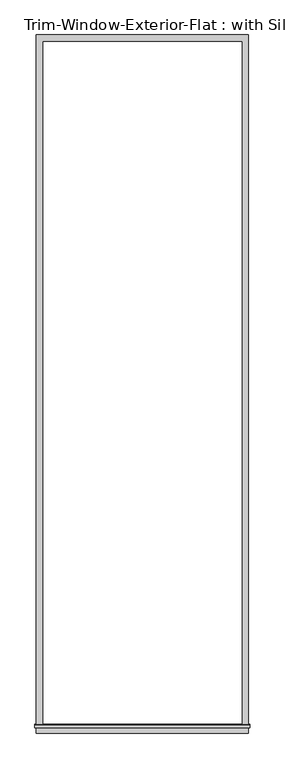
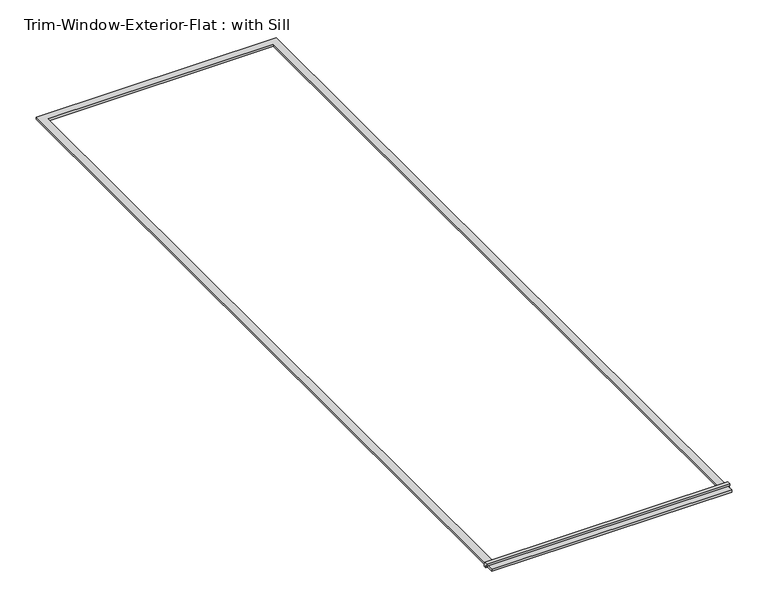
"""IFC4 building model written with IfcOpenShell, lengths in millimetres: proxy geometry, Trim-Window-Exterior-Flat : with Sill."""

from ifc_helpers import new_model, si_unit, frame, origin, origin_with_axes, place, context, project, spatial, polyline, outline, extrude, source, transform, mapped, element, save


def trim_window_exterior_flat_with_sill_953729a5(model_context):
    return source(origin(), model_context, "Body", "SweptSolid", [
        extrude(outline(polyline([(971.55, -6270.5823709), (971.55, -6327.7323709), (-971.55, -6327.7323709), (-971.55, -6270.5823709), (971.55, -6270.5823709)])), origin_with_axes(), (0.0, 0.0, 1.0), 19.05),
        extrude(outline(polyline([(-6280.15, 38.1), (-6250.8580645, 38.1), (-6248.4, 19.05), (-6248.4, 0.0), (-6270.5823709, 0.0), (-6270.5823709, 19.05), (-6280.15, 19.05), (-6280.15, 38.1)])), frame((-984.25, 0.0, 0.0), z_axis=(1.0, 0.0, 0.0), x_axis=(0.0, 1.0, 0.0)), (0.0, 0.0, 1.0), 1968.5),
        extrude(outline(polyline([(-971.55, 57.15), (971.55, 57.15), (971.55, -6248.4), (914.4, -6248.4), (914.4, 0.0), (-914.4, 0.0), (-914.4, -6248.4), (-971.55, -6248.4), (-971.55, 57.15)])), origin_with_axes(), (0.0, 0.0, 1.0), 19.05),
    ])


if __name__ == "__main__":
    model = new_model("IFC4")
    model_context = context("Model", 3, world=origin())
    ifc_project = project(units=[si_unit("LENGTHUNIT", "METRE", prefix="MILLI")], contexts=[model_context])
    site = spatial("IfcSite", under=ifc_project)
    building = spatial("IfcBuilding", under=site)
    placement = place(None, origin())
    trim_window_exterior_flat_with_sill_shape = trim_window_exterior_flat_with_sill_953729a5(model_context)
    element("IfcBuildingElementProxy", 1, Name="Trim-Window-Exterior-Flat : with Sill", ObjectType="Trim-Window-Exterior-Flat : with Sill", at=placement, inside=building, context=model_context, shape_type="MappedRepresentation", body=[
        mapped(trim_window_exterior_flat_with_sill_shape, transform((0.0, 0.0, 0.0), x_axis=(1.0, 0.0, 0.0), y_axis=(0.0, 1.0, 0.0), z_axis=(0.0, 0.0, 1.0))),
    ])
    save(model, "model.ifc")

# Revit data of these elements
# Type "Trim-Window-Exterior-Flat : with Sill"
#   Trim Width = 0' - 2 1/4"
#   Trim Thickness_Picture Frame = 0' - 1 1/4"
#   Trim Thickness_with Sill = 0' - 0 3/4"
#   Sill Thickness = 0' - 1 1/4"
#   Opening Width [instance default] = 2' - 0"
#   Opening Height [instance default] = 3' - 0"
#   Default Elevation = 4' - 0"
#   Sill = yes
#   Picture Frame = no
#   Trim Material [instance default] = none
# Element 1 (IfcBuildingElementProxy, "Trim-Window-Exterior-Flat : with Sill")
#   Opening Width = 6' - 0"
#   Opening Height = 20' - 6"
#   Trim Material = Clad - White
#   Materials on its faces: "Clad - White"
# Materials
#   "Clad - White": class "Wood", colour RGB 242 242 238, transparency 0, Cost = 0
